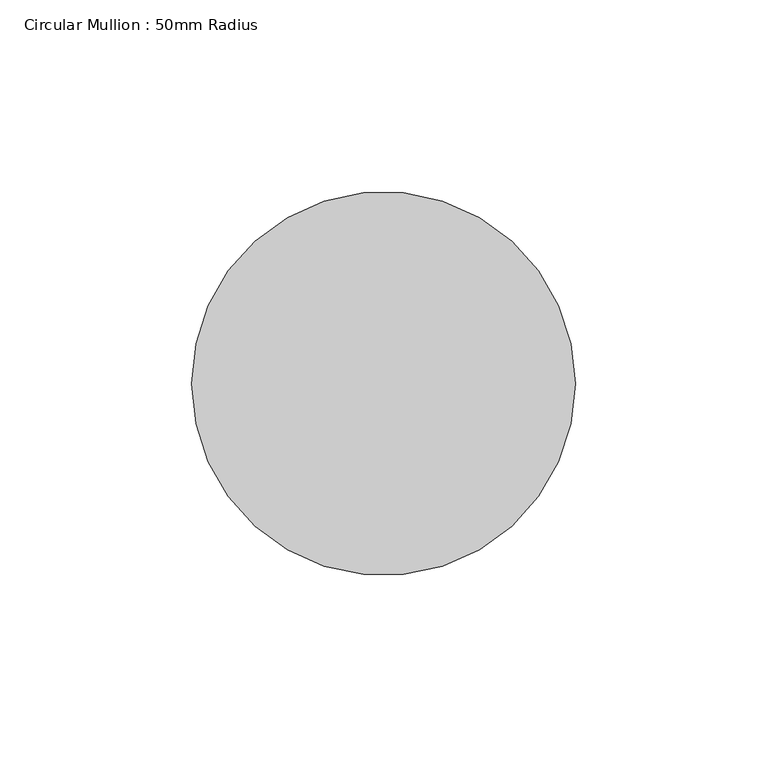
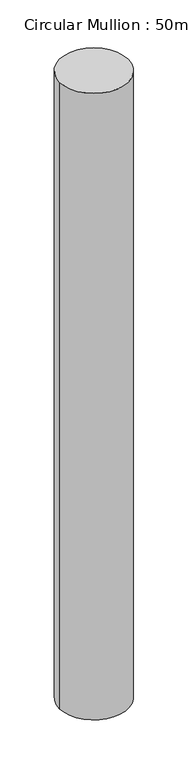
"""IFC4 building model written with IfcOpenShell, lengths in millimetres: member geometry, Circular Mullion : 50mm Radius."""

from ifc_helpers import new_model, si_unit, point, frame, origin, origin_2d, place, context, project, spatial, circle_curve, trimmed, segment, composite_curve, outline, extrude, source, transform, mapped, element, save


def circular_mullion_50mm_radius_698fe6c3(model_context):
    return source(origin(), model_context, "Body", "SweptSolid", [
        extrude(outline(composite_curve([segment(trimmed(circle_curve(origin_2d(), 50.0), [point((50.0, 0.0))], [point((-50.0, 0.0))], False, "CARTESIAN"), True, "CONTINUOUS"), segment(trimmed(circle_curve(origin_2d(), 50.0), [point((-50.0, 0.0))], [point((50.0, 0.0))], False, "CARTESIAN"), True, "CONTINUOUS")], self_intersect=False)), frame((0.0, 0.0, -964.2348478), z_axis=(0.0, 0.0, 1.0), x_axis=(1.0, 0.0, 0.0)), (0.0, 0.0, 1.0), 964.2348478),
    ])


if __name__ == "__main__":
    model = new_model("IFC4")
    model_context = context("Model", 3, world=origin())
    ifc_project = project(units=[si_unit("LENGTHUNIT", "METRE", prefix="MILLI")], contexts=[model_context])
    site = spatial("IfcSite", under=ifc_project)
    building = spatial("IfcBuilding", under=site)
    placement = place(None, origin())
    circular_mullion_50mm_radius_shape = circular_mullion_50mm_radius_698fe6c3(model_context)
    element("IfcMember", 1, ObjectType="Circular Mullion : 50mm Radius", at=placement, inside=building, context=model_context, shape_type="MappedRepresentation", body=[
        mapped(circular_mullion_50mm_radius_shape, transform((0.0, 0.0, 0.0), x_axis=(1.0, 0.0, 0.0), y_axis=(0.0, 1.0, 0.0), z_axis=(0.0, 0.0, 1.0))),
    ])
    save(model, "model.ifc")

# Revit data of these elements
# Type "Circular Mullion : 50mm Radius"
#   built-in parameter 1007350 = 0.164042 (stored number, unit not read)
# Element 1 (IfcMember, "Circular Mullion : 50mm Radius")
#   Materials on its faces: "Aluminium"
# Materials
#   "Aluminium": class "Metal", colour RGB 247 247 247, transparency 0, Description = "Aluminium 6061", Cost = 0
